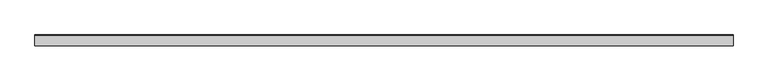
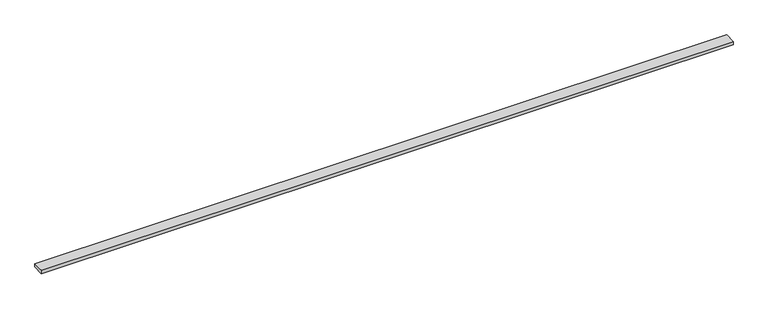
"""IFC4 building model written with IfcOpenShell, lengths in millimetres: proxy geometry, Inner panel:Inner panel:1:Inner panel:1 : Inner panel:Inner panel:300324:2:Inner panel:1:Inner panel:1 : Inner panel:Inner panel:300324:2 : Inner panel:Inner panel:1:Inner panel:1 : Inner panel:Inner panel:300324:300043:40 : Inner panel:Inner panel:1:Inner panel:1 : Inner panel:Inner panel:300324:2:Inner panel:1:Inner panel:1 : Inner panel:Inner panel:300324:2 : Inner panel:Inner panel:1:Inner panel:1 : Inner panel:Inner panel:300324:300043:308120."""

from ifc_helpers import new_model, si_unit, frame, origin, place, context, project, spatial, polyline, outline, extrude, source, transform, mapped, element, save


def generic_models_594c6d27(model_context):
    return source(origin(), model_context, "Body", "SweptSolid", [
        extrude(outline(polyline([(0.0, -75.8934963), (0.0, 0.0), (4876.8, 0.0), (4876.8, -75.8934963), (0.0, -75.8934963)])), frame((615791.6367239, -576391.370927, 4033.1979981), z_axis=(0.0, -0.04163054471215047, 0.9991330730923532), x_axis=(-1.0, 0.0, 0.0)), (0.0, 0.0, 1.0), 25.4),
    ])


if __name__ == "__main__":
    model = new_model("IFC4")
    model_context = context("Model", 3, world=origin())
    ifc_project = project(units=[si_unit("LENGTHUNIT", "METRE", prefix="MILLI")], contexts=[model_context])
    site = spatial("IfcSite", under=ifc_project)
    building = spatial("IfcBuilding", under=site)
    placement = place(None, origin())
    generic_models_shape = generic_models_594c6d27(model_context)
    element("IfcBuildingElementProxy", 1, Name="Inner panel:Inner panel:1:Inner panel:1 : Inner panel:Inner panel:300324:2:Inner panel:1:Inner panel:1 : Inner panel:Inner panel:300324:2 : Inner panel:Inner panel:1:Inner panel:1 : Inner panel:Inner panel:300324:300043:40 : Inner panel:Inner panel:1:Inner panel:1 : Inner panel:Inner panel:300324:2:Inner panel:1:Inner panel:1 : Inner panel:Inner panel:300324:2 : Inner panel:Inner panel:1:Inner panel:1 : Inner panel:Inner panel:300324:300043:308120", ObjectType="Inner panel:Inner panel:1:Inner panel:1 : Inner panel:Inner panel:300324:2:Inner panel:1:Inner panel:1 : Inner panel:Inner panel:300324:2 : Inner panel:Inner panel:1:Inner panel:1 : Inner panel:Inner panel:300324:300043:40 : Inner panel:Inner panel:1:Inner panel:1 : Inner panel:Inner panel:300324:2:Inner panel:1:Inner panel:1 : Inner panel:Inner panel:300324:2 : Inner panel:Inner panel:1:Inner panel:1 : Inner panel:Inner panel:300324:300043:308120", at=placement, inside=building, context=model_context, shape_type="MappedRepresentation", body=[
        mapped(generic_models_shape, transform((0.0, 0.0, 0.0), x_axis=(1.0, 0.0, 0.0), y_axis=(0.0, 1.0, 0.0), z_axis=(0.0, 0.0, 1.0))),
    ])
    save(model, "model.ifc")

# Revit data of these elements
# Type "Inner panel:Inner panel:1:Inner panel:1 : Inner panel:Inner panel:300324:2:Inner panel:1:Inner panel:1 : Inner panel:Inner panel:300324:2 : Inner panel:Inner panel:1:Inner panel:1 : Inner panel:Inner panel:300324:300043:40 : Inner panel:Inner panel:1:Inner panel:1 : Inner panel:Inner panel:300324:2:Inner panel:1:Inner panel:1 : Inner panel:Inner panel:300324:2 : Inner panel:Inner panel:1:Inner panel:1 : Inner panel:Inner panel:300324:300043:308120"
#   NameOverride = "Inner panel:Inner panel:1:Inner panel:1 : Inner panel:Inner panel:300324:2:Inner panel:1:Inner panel:1 : Inner panel:Inner panel:300324:2 : Inner panel:Inner panel:1:Inner panel:1 : Inner panel:Inner panel:300324:300043:308120"
#   ObjectTypeOverride = "Inner panel:1:Inner panel:1 : Inner panel:Inner panel:300324:2 : Inner panel:Inner panel:1:Inner panel:1 : Inner panel:Inner panel:300324:300043"
#   Reference = "Inner panel"
#   Tag = "308120"
# Element 1 (IfcBuildingElementProxy, "Inner panel:Inner panel:1:Inner panel:1 : Inner panel:Inner panel:300324:2:Inner panel:1:Inner panel:1 : Inner panel:Inner panel:300324:2 : Inner panel:Inner panel:1:Inner panel:1 : Inner panel:Inner panel:300324:300043:40 : Inner panel:Inner panel:1:Inner panel:1 : Inner panel:Inner panel:300324:2:Inner panel:1:Inner panel:1 : Inner panel:Inner panel:300324:2 : Inner panel:Inner panel:1:Inner panel:1 : Inner panel:Inner panel:300324:300043:308120")
#   Materials on its faces: "1\" THERMAL SPACER @ PURLIN"
# Materials
#   "1\" THERMAL SPACER @ PURLIN": class "Unassigned", colour RGB 205 188 106, transparency 0, Cost = 0
